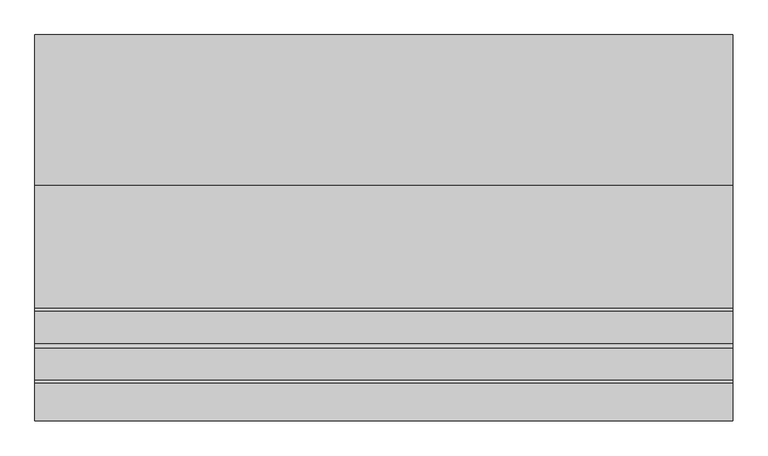
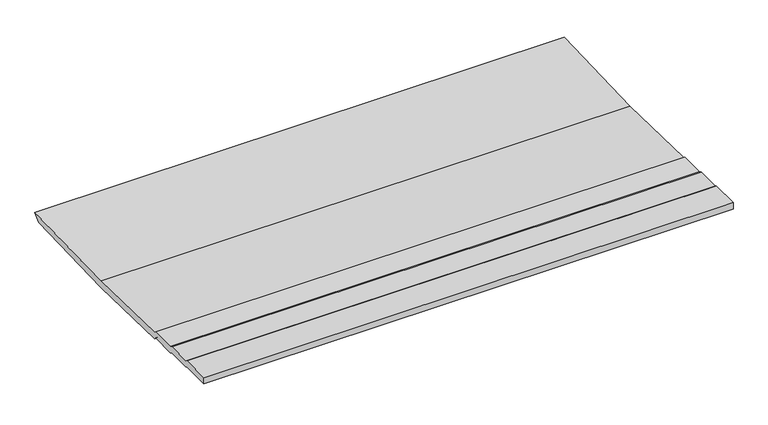
"""IFC4 building model written with IfcOpenShell, lengths in millimetres: proxy geometry, GRAVEL BALLAST002 34887 : GRAVEL BALLAST002 34887."""

import ifcopenshell
import ifcopenshell.guid

model = None  # the IFC model being written
_history = None  # IfcOwnerHistory: only IFC2X3 demands one
_inside = {}  # id of a spatial element -> (the spatial element, [elements in it])
_under = {}  # id of a project, library or spatial element -> (it, [spatial elements below it])
_declared = {}  # id of a project -> (the project, [libraries it declares])
_typed = {}  # id of a type object -> (the type object, [elements of that type])
_made_of = {}  # id of a material, layer set ... -> (it, [elements and type objects made of it])


def new_model(schema):
    """Start an empty IFC model of exactly this schema.

    Asked for "IFC4X3", IfcOpenShell would pick the latest addendum, in which some entities
    have other attributes; the version numbers below select the first issue.
    IFC2X3 requires an IfcOwnerHistory on every rooted entity: one is made here for all.
    """
    global model, _history
    if schema == "IFC4X3":
        model = ifcopenshell.file(schema_version=(4, 3, 0, 0))
    else:
        model = ifcopenshell.file(schema=schema)
    _inside.clear()
    _under.clear()
    _declared.clear()
    _typed.clear()
    _made_of.clear()
    _history = None
    if model.schema == "IFC2X3":
        org = make("IfcOrganization", Name="unknown")
        user = make(
            "IfcPersonAndOrganization",
            ThePerson=make("IfcPerson", FamilyName="unknown"),
            TheOrganization=org,
        )
        app = make(
            "IfcApplication",
            ApplicationDeveloper=org,
            Version="unknown",
            ApplicationFullName="unknown",
            ApplicationIdentifier="unknown",
        )
        _history = make(
            "IfcOwnerHistory",
            OwningUser=user,
            OwningApplication=app,
            ChangeAction="ADDED",
            CreationDate=0,
        )
    return model


def make(cls, **values):
    """One entity of the class cls with the attributes given. An attribute that is None is left unset."""
    return model.create_entity(
        cls, **{name: value for name, value in values.items() if value is not None}
    )


def rooted(cls, **values):
    """An entity with a GlobalId (a new one), such as an element, a storey or a relation."""
    return make(cls, GlobalId=ifcopenshell.guid.new(), OwnerHistory=_history, **values)


def si_unit(unit_type, name, prefix=None):
    """IfcSIUnit, for example si_unit("LENGTHUNIT", "METRE", prefix="MILLI")."""
    return make("IfcSIUnit", UnitType=unit_type, Prefix=prefix, Name=name)


def assignment(units):
    """IfcUnitAssignment: the units of a project."""
    return None if units is None else make("IfcUnitAssignment", Units=units)


def point(xyz):
    """IfcCartesianPoint."""
    return None if xyz is None else make("IfcCartesianPoint", Coordinates=xyz)


def direction(xyz):
    """IfcDirection."""
    return None if xyz is None else make("IfcDirection", DirectionRatios=xyz)


def frame(location, z_axis=None, x_axis=None):
    """IfcAxis2Placement3D, a coordinate frame: its origin and axes. An axis left out is left unset."""
    return make(
        "IfcAxis2Placement3D",
        Location=point(location),
        Axis=direction(z_axis),
        RefDirection=direction(x_axis),
    )


def origin():
    """The frame at (0, 0, 0) with its axes left unset."""
    return frame((0.0, 0.0, 0.0))


def place(relative_to, where):
    """IfcLocalPlacement: puts the frame where relative to a parent placement (None: the world)."""
    return make(
        "IfcLocalPlacement", PlacementRelTo=relative_to, RelativePlacement=where
    )


def context(
    kind, dimensions, precision=None, world=None, true_north=None, identifier=None
):
    """IfcGeometricRepresentationContext, for example the 3D "Model" context."""
    return make(
        "IfcGeometricRepresentationContext",
        ContextIdentifier=identifier,
        ContextType=kind,
        CoordinateSpaceDimension=dimensions,
        Precision=precision,
        WorldCoordinateSystem=world,
        TrueNorth=true_north,
    )


def project(units=None, contexts=None):
    """IfcProject with its units and contexts."""
    return rooted(
        "IfcProject",
        Name="project",
        RepresentationContexts=contexts,
        UnitsInContext=assignment(units),
    )


def spatial(cls, under=None, at=None, **own):
    """A site, building, storey or space (cls), placed at a placement, below another one or the project."""
    s = rooted(cls, ObjectPlacement=at, **own)
    if under is not None:
        _under.setdefault(under.id(), (under, []))[1].append(s)
    return s


def polyline(points):
    """IfcPolyline through the points."""
    return make("IfcPolyline", Points=[point(p) for p in points])


def outline(outer, holes=None, kind="AREA"):
    """IfcArbitraryClosedProfileDef: a profile drawn as a closed curve; with holes, ...WithVoids."""
    if holes is None:
        return make("IfcArbitraryClosedProfileDef", ProfileType=kind, OuterCurve=outer)
    return make(
        "IfcArbitraryProfileDefWithVoids",
        ProfileType=kind,
        OuterCurve=outer,
        InnerCurves=holes,
    )


def extrude(swept, where, along, depth):
    """IfcExtrudedAreaSolid: the profile swept, set in the frame where, extruded along a direction by depth."""
    return make(
        "IfcExtrudedAreaSolid",
        SweptArea=swept,
        Position=where,
        ExtrudedDirection=direction(along),
        Depth=depth,
    )


def shape(context_of_items, identifier, shape_type, items):
    """IfcShapeRepresentation: the items that make up one representation, for example the "Body"."""
    return make(
        "IfcShapeRepresentation",
        ContextOfItems=context_of_items,
        RepresentationIdentifier=identifier,
        RepresentationType=shape_type,
        Items=items,
    )


def source(mapping_origin, context_of_items, identifier, shape_type, items):
    """IfcRepresentationMap: a shape defined once, which mapped items show again and again."""
    return make(
        "IfcRepresentationMap",
        MappingOrigin=mapping_origin,
        MappedRepresentation=shape(context_of_items, identifier, shape_type, items),
    )


def transform(
    local_origin,
    x_axis=None,
    y_axis=None,
    z_axis=None,
    scale=None,
    scale2=None,
    scale3=None,
    uniform=True,
):
    """IfcCartesianTransformationOperator3D, or its non-uniform kind. x_axis, y_axis, z_axis: its Axis1, 2, 3."""
    if uniform:
        return make(
            "IfcCartesianTransformationOperator3D",
            Axis1=direction(x_axis),
            Axis2=direction(y_axis),
            LocalOrigin=point(local_origin),
            Scale=scale,
            Axis3=direction(z_axis),
        )
    return make(
        "IfcCartesianTransformationOperator3DnonUniform",
        Axis1=direction(x_axis),
        Axis2=direction(y_axis),
        LocalOrigin=point(local_origin),
        Scale=scale,
        Axis3=direction(z_axis),
        Scale2=scale2,
        Scale3=scale3,
    )


def mapped(mapping_source, mapping_target):
    """IfcMappedItem: shows the shape of a source again, moved by a transform."""
    return make(
        "IfcMappedItem", MappingSource=mapping_source, MappingTarget=mapping_target
    )


def made_of(thing, what):
    """Note that an element or type object is made of a material, layer set ...; save() writes the relation."""
    if what is not None:
        _made_of.setdefault(what.id(), (what, []))[1].append(thing)
    return thing


def element(
    cls,
    number,
    at=None,
    inside=None,
    cuts=None,
    type_object=None,
    material=None,
    context=None,
    identifier="Body",
    shape_type=None,
    held_by="IfcProductDefinitionShape",
    body=None,
    shapes=None,
    **own,
):
    """One element of the class cls, such as IfcWall. Its Tag is "e" and its number.

    at: its placement. inside: the storey or other place that contains it. cuts: it is an
    opening in that element (IfcRelVoidsElement). A single representation is given by context,
    identifier, shape_type and body (its items); several are given by shapes. held_by: the class
    of the entity that holds the representations. save() writes the other relations.
    """
    e = rooted(cls, Tag="e%d" % number, ObjectPlacement=at, **own)
    if body is not None:
        shapes = [shape(context, identifier, shape_type, body)]
    if shapes is not None:
        e.Representation = make(held_by, Representations=shapes)
    if inside is not None:
        _inside.setdefault(inside.id(), (inside, []))[1].append(e)
    if cuts is not None:
        rooted(
            "IfcRelVoidsElement", RelatingBuildingElement=cuts, RelatedOpeningElement=e
        )
    if type_object is not None:
        _typed.setdefault(type_object.id(), (type_object, []))[1].append(e)
    return made_of(e, material)


def aggregate(whole, parts):
    """IfcRelAggregates: a whole, such as a stair, and the parts it consists of."""
    return rooted("IfcRelAggregates", RelatingObject=whole, RelatedObjects=parts)


def save(model, path):
    """Write the relations noted so far, then the file.

    IfcRelAggregates (storeys below a building ...), IfcRelContainedInSpatialStructure (elements
    in a storey), IfcRelDefinesByType, IfcRelAssociatesMaterial and IfcRelDeclares: one each for
    every whole, place, type object, material and project.
    """
    for whole, parts in _under.values():
        aggregate(whole, parts)
    for where, things in _inside.values():
        rooted(
            "IfcRelContainedInSpatialStructure",
            RelatedElements=things,
            RelatingStructure=where,
        )
    for kind, things in _typed.values():
        rooted("IfcRelDefinesByType", RelatedObjects=things, RelatingType=kind)
    for what, things in _made_of.values():
        rooted("IfcRelAssociatesMaterial", RelatedObjects=things, RelatingMaterial=what)
    for by, libraries in _declared.values():
        rooted("IfcRelDeclares", RelatingContext=by, RelatedDefinitions=libraries)
    model.write(path)


def generic_models_c19f6b3d(model_context):
    return source(origin(), model_context, "Body", "SweptSolid", [
        extrude(outline(polyline([(-5440.365918, 40253.79375), (-5549.8654297, 40253.79375), (-5549.8654297, 40278.5320313), (-5440.365918, 40278.5320313), (-5431.6554687, 40274.2507813), (-5341.0685547, 40274.2507813), (-5328.2239153, 40268.5233193), (-5234.272168, 40270.16875), (-5225.9987305, 40262.7585938), (-4873.4420898, 40254.5398438), (-4442.8393555, 40268.1982422), (-4468.0649414, 40242.9726562), (-4873.4420898, 40229.8015625), (-5225.9987305, 40238.0203125), (-5234.272168, 40245.4304687), (-5328.2239153, 40243.785038), (-5341.0685547, 40249.5125), (-5431.6554687, 40249.5125), (-5440.365918, 40253.79375)])), frame((12382.7678845, 0.0, 0.0), z_axis=(1.0, 0.0, 0.0), x_axis=(0.0, 1.0, 0.0)), (0.0, 0.0, 1.0), 2000.0),
    ])


if __name__ == "__main__":
    model = new_model("IFC4")
    model_context = context("Model", 3, world=origin())
    ifc_project = project(units=[si_unit("LENGTHUNIT", "METRE", prefix="MILLI")], contexts=[model_context])
    site = spatial("IfcSite", under=ifc_project)
    building = spatial("IfcBuilding", under=site)
    placement = place(None, origin())
    generic_models_shape = generic_models_c19f6b3d(model_context)
    element("IfcBuildingElementProxy", 1, Name="GRAVEL BALLAST002 34887 : GRAVEL BALLAST002 34887", ObjectType="GRAVEL BALLAST002 34887 : GRAVEL BALLAST002 34887", at=placement, inside=building, context=model_context, shape_type="MappedRepresentation", body=[
        mapped(generic_models_shape, transform((0.0, 0.0, 0.0), x_axis=(1.0, 0.0, 0.0), y_axis=(0.0, 1.0, 0.0), z_axis=(0.0, 0.0, 1.0))),
    ])
    save(model, "model.ifc")

# Revit data of these elements
# Type "GRAVEL BALLAST002 34887 : GRAVEL BALLAST002 34887"
#   NameOverride = "GRAVEL BALLAST002"
# Element 1 (IfcBuildingElementProxy, "GRAVEL BALLAST002 34887 : GRAVEL BALLAST002 34887")
#   Materials on its faces: "GRAVEL BALLAST"
# Materials
#   "GRAVEL BALLAST": class "Unassigned", colour RGB 128 128 128, transparency 0, Cost = 0
